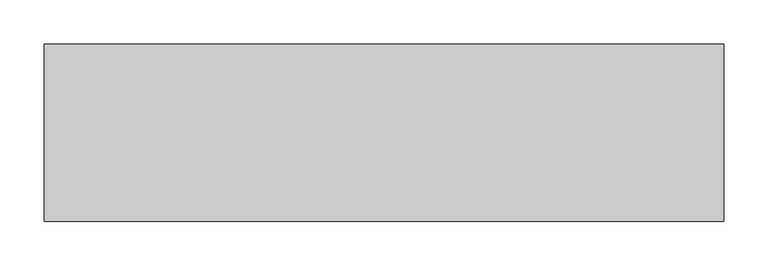
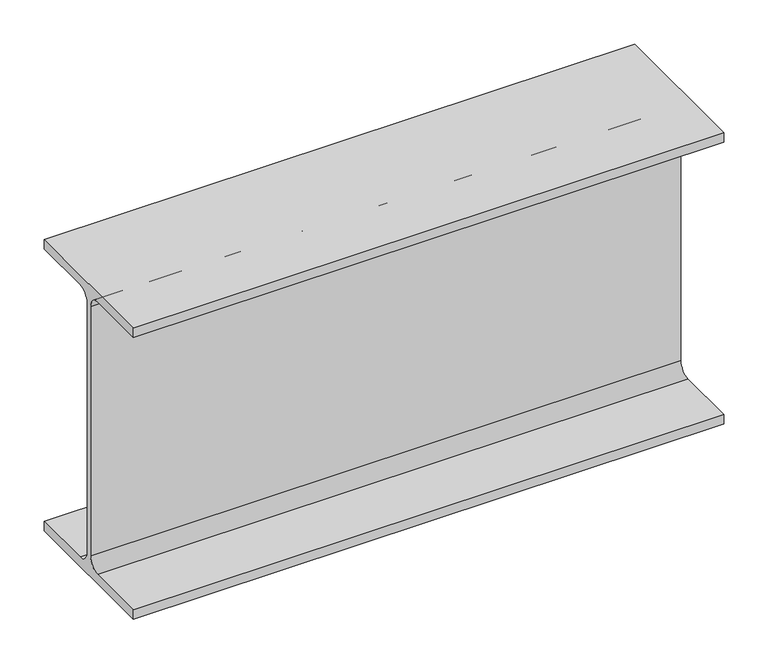
"""IFC4 building model written with IfcOpenShell, lengths in millimetres: beam geometry, Steel Framing_H_KS : H_SB_AR_S02_H-400x200x8x13_SCB1."""

from ifc_helpers import new_model, si_unit, point, frame, frame_2d, origin, place, context, project, spatial, polyline, circle_curve, trimmed, segment, composite_curve, outline, extrude, source, transform, mapped, element, save


def beam_a081c7c9(model_context):
    return source(origin(), model_context, "Body", "SweptSolid", [
        extrude(outline(composite_curve([segment(polyline([(100.0, -187.0), (100.0, -200.0), (-100.0, -200.0), (-100.0, -187.0), (-20.0, -187.0)]), True, "CONTINUOUS"), segment(trimmed(circle_curve(frame_2d((-20.0, -171.0)), 16.0), [point((-20.0, -187.0))], [point((-4.0, -171.0))], True, "CARTESIAN"), True, "CONTINUOUS"), segment(polyline([(-4.0, -171.0), (-4.0, 171.0)]), True, "CONTINUOUS"), segment(trimmed(circle_curve(frame_2d((-20.0, 171.0)), 16.0), [point((-4.0, 171.0))], [point((-20.0, 187.0))], True, "CARTESIAN"), True, "CONTINUOUS"), segment(polyline([(-20.0, 187.0), (-100.0, 187.0), (-100.0, 200.0), (100.0, 200.0), (100.0, 187.0), (20.0, 187.0)]), True, "CONTINUOUS"), segment(trimmed(circle_curve(frame_2d((20.0, 171.0)), 16.0), [point((20.0, 187.0))], [point((4.0, 171.0))], True, "CARTESIAN"), True, "CONTINUOUS"), segment(polyline([(4.0, 171.0), (4.0, -171.0)]), True, "CONTINUOUS"), segment(trimmed(circle_curve(frame_2d((20.0, -171.0)), 16.0), [point((4.0, -171.0))], [point((20.0, -187.0))], True, "CARTESIAN"), True, "CONTINUOUS"), segment(polyline([(20.0, -187.0), (100.0, -187.0)]), True, "CONTINUOUS")], self_intersect=False)), frame((-236.0, 0.0, 0.0), z_axis=(1.0, 0.0, 0.0), x_axis=(0.0, 1.0, 0.0)), (0.0, 0.0, 1.0), 766.0),
    ])


if __name__ == "__main__":
    model = new_model("IFC4")
    model_context = context("Model", 3, world=origin())
    ifc_project = project(units=[si_unit("LENGTHUNIT", "METRE", prefix="MILLI")], contexts=[model_context])
    site = spatial("IfcSite", under=ifc_project)
    building = spatial("IfcBuilding", under=site)
    placement = place(None, origin())
    beam_shape = beam_a081c7c9(model_context)
    element("IfcBeam", 1, ObjectType="Steel Framing_H_KS : H_SB_AR_S02_H-400x200x8x13_SCB1", at=placement, inside=building, context=model_context, shape_type="MappedRepresentation", body=[
        mapped(beam_shape, transform((0.0, 0.0, 0.0), x_axis=(1.0, 0.0, 0.0), y_axis=(0.0, 1.0, 0.0), z_axis=(0.0, 0.0, 1.0))),
    ])
    save(model, "model.ifc")

# Revit data of these elements
# Type "Steel Framing_H_KS : H_SB_AR_S02_H-400x200x8x13_SCB1"
#   Type Comments = "MAIN"
#   Type Mark = "SCB1"
#   H_SectionID = "H-400x200x8x13"
#   H_Ratio for Additional Steel Plate = 0.2
#   Width = 20.0 cm
#   Web Thickness = 0.8 cm
#   Web Fillet = 1.6 cm
#   Warping Constant = 649000.0 cm⁶
#   Torsional Moment of Inertia = 35.8981 cm⁴
#   Section Area = 84.12 cm²
#   Plastic Modulus weak axis = 268.0 cm³
#   Plastic Modulus strong axis = 1330.0 cm³
#   Perimeter = 1.56 m²/m
#   Nominal Weight = 66.00 kgf/m
#   Moment of Inertia weak axis = 1740.00 cm⁴
#   Moment of Inertia strong axis = 23700.00 cm⁴
#   Height = 40.0 cm
#   Flange Thickness = 1.3 cm
#   Elastic Modulus weak axis = 174.0 cm³
#   Elastic Modulus strong axis = 1190.0 cm³
#   Centroid Vertical = 20.0 cm
#   Centroid Horizontal = 10.0 cm
#   Bolt Spacing = 8.89 cm
#   Length [instance default] = 1500 mm
#   Structural Material [instance default] = Steel, 45-345
#   Section Name Key = ""
#   Assembly Code = ""
# Element 1 (IfcBeam, "Steel Framing_H_KS : H_SB_AR_S02_H-400x200x8x13_SCB1")
#   Materials on its faces: "Steel, 45-345"
# Materials
#   "Steel, 45-345": class "Metal", colour RGB 189 187 185, transparency 0, Description = "Steel 345 MPa", Cost = 0
